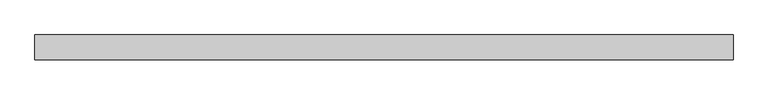
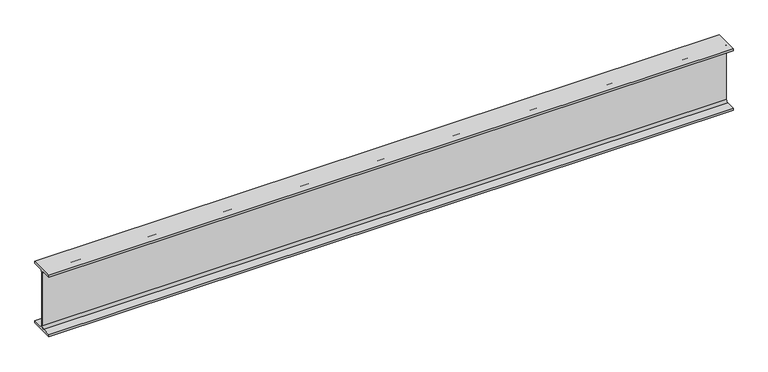
"""IFC4 building model written with IfcOpenShell, lengths in millimetres: beam geometry, 0912_Steel Framing_H-KSD3502 : H_SB_ASB_H-800x300x14x26."""

import ifcopenshell
import ifcopenshell.guid

model = None  # the IFC model being written
_history = None  # IfcOwnerHistory: only IFC2X3 demands one
_inside = {}  # id of a spatial element -> (the spatial element, [elements in it])
_under = {}  # id of a project, library or spatial element -> (it, [spatial elements below it])
_declared = {}  # id of a project -> (the project, [libraries it declares])
_typed = {}  # id of a type object -> (the type object, [elements of that type])
_made_of = {}  # id of a material, layer set ... -> (it, [elements and type objects made of it])


def new_model(schema):
    """Start an empty IFC model of exactly this schema.

    Asked for "IFC4X3", IfcOpenShell would pick the latest addendum, in which some entities
    have other attributes; the version numbers below select the first issue.
    IFC2X3 requires an IfcOwnerHistory on every rooted entity: one is made here for all.
    """
    global model, _history
    if schema == "IFC4X3":
        model = ifcopenshell.file(schema_version=(4, 3, 0, 0))
    else:
        model = ifcopenshell.file(schema=schema)
    _inside.clear()
    _under.clear()
    _declared.clear()
    _typed.clear()
    _made_of.clear()
    _history = None
    if model.schema == "IFC2X3":
        org = make("IfcOrganization", Name="unknown")
        user = make(
            "IfcPersonAndOrganization",
            ThePerson=make("IfcPerson", FamilyName="unknown"),
            TheOrganization=org,
        )
        app = make(
            "IfcApplication",
            ApplicationDeveloper=org,
            Version="unknown",
            ApplicationFullName="unknown",
            ApplicationIdentifier="unknown",
        )
        _history = make(
            "IfcOwnerHistory",
            OwningUser=user,
            OwningApplication=app,
            ChangeAction="ADDED",
            CreationDate=0,
        )
    return model


def make(cls, **values):
    """One entity of the class cls with the attributes given. An attribute that is None is left unset."""
    return model.create_entity(
        cls, **{name: value for name, value in values.items() if value is not None}
    )


def rooted(cls, **values):
    """An entity with a GlobalId (a new one), such as an element, a storey or a relation."""
    return make(cls, GlobalId=ifcopenshell.guid.new(), OwnerHistory=_history, **values)


def si_unit(unit_type, name, prefix=None):
    """IfcSIUnit, for example si_unit("LENGTHUNIT", "METRE", prefix="MILLI")."""
    return make("IfcSIUnit", UnitType=unit_type, Prefix=prefix, Name=name)


def assignment(units):
    """IfcUnitAssignment: the units of a project."""
    return None if units is None else make("IfcUnitAssignment", Units=units)


def point(xyz):
    """IfcCartesianPoint."""
    return None if xyz is None else make("IfcCartesianPoint", Coordinates=xyz)


def direction(xyz):
    """IfcDirection."""
    return None if xyz is None else make("IfcDirection", DirectionRatios=xyz)


def frame(location, z_axis=None, x_axis=None):
    """IfcAxis2Placement3D, a coordinate frame: its origin and axes. An axis left out is left unset."""
    return make(
        "IfcAxis2Placement3D",
        Location=point(location),
        Axis=direction(z_axis),
        RefDirection=direction(x_axis),
    )


def frame_2d(location, x_axis=None):
    """IfcAxis2Placement2D, a coordinate frame in the plane: its origin and x axis."""
    return make(
        "IfcAxis2Placement2D", Location=point(location), RefDirection=direction(x_axis)
    )


def origin():
    """The frame at (0, 0, 0) with its axes left unset."""
    return frame((0.0, 0.0, 0.0))


def place(relative_to, where):
    """IfcLocalPlacement: puts the frame where relative to a parent placement (None: the world)."""
    return make(
        "IfcLocalPlacement", PlacementRelTo=relative_to, RelativePlacement=where
    )


def context(
    kind, dimensions, precision=None, world=None, true_north=None, identifier=None
):
    """IfcGeometricRepresentationContext, for example the 3D "Model" context."""
    return make(
        "IfcGeometricRepresentationContext",
        ContextIdentifier=identifier,
        ContextType=kind,
        CoordinateSpaceDimension=dimensions,
        Precision=precision,
        WorldCoordinateSystem=world,
        TrueNorth=true_north,
    )


def project(units=None, contexts=None):
    """IfcProject with its units and contexts."""
    return rooted(
        "IfcProject",
        Name="project",
        RepresentationContexts=contexts,
        UnitsInContext=assignment(units),
    )


def spatial(cls, under=None, at=None, **own):
    """A site, building, storey or space (cls), placed at a placement, below another one or the project."""
    s = rooted(cls, ObjectPlacement=at, **own)
    if under is not None:
        _under.setdefault(under.id(), (under, []))[1].append(s)
    return s


def polyline(points):
    """IfcPolyline through the points."""
    return make("IfcPolyline", Points=[point(p) for p in points])


def circle_curve(where, radius):
    """IfcCircle in the frame where."""
    return make("IfcCircle", Position=where, Radius=radius)


def trimmed(basis, trim1, trim2, sense, master):
    """IfcTrimmedCurve: the piece of a basis curve between two trims."""
    return make(
        "IfcTrimmedCurve",
        BasisCurve=basis,
        Trim1=trim1,
        Trim2=trim2,
        SenseAgreement=sense,
        MasterRepresentation=master,
    )


def segment(curve, same_sense, transition):
    """IfcCompositeCurveSegment."""
    return make(
        "IfcCompositeCurveSegment",
        Transition=transition,
        SameSense=same_sense,
        ParentCurve=curve,
    )


def composite_curve(segments, self_intersect=None):
    """IfcCompositeCurve: segments joined end to end."""
    return make("IfcCompositeCurve", Segments=segments, SelfIntersect=self_intersect)


def outline(outer, holes=None, kind="AREA"):
    """IfcArbitraryClosedProfileDef: a profile drawn as a closed curve; with holes, ...WithVoids."""
    if holes is None:
        return make("IfcArbitraryClosedProfileDef", ProfileType=kind, OuterCurve=outer)
    return make(
        "IfcArbitraryProfileDefWithVoids",
        ProfileType=kind,
        OuterCurve=outer,
        InnerCurves=holes,
    )


def extrude(swept, where, along, depth):
    """IfcExtrudedAreaSolid: the profile swept, set in the frame where, extruded along a direction by depth."""
    return make(
        "IfcExtrudedAreaSolid",
        SweptArea=swept,
        Position=where,
        ExtrudedDirection=direction(along),
        Depth=depth,
    )


def shape(context_of_items, identifier, shape_type, items):
    """IfcShapeRepresentation: the items that make up one representation, for example the "Body"."""
    return make(
        "IfcShapeRepresentation",
        ContextOfItems=context_of_items,
        RepresentationIdentifier=identifier,
        RepresentationType=shape_type,
        Items=items,
    )


def source(mapping_origin, context_of_items, identifier, shape_type, items):
    """IfcRepresentationMap: a shape defined once, which mapped items show again and again."""
    return make(
        "IfcRepresentationMap",
        MappingOrigin=mapping_origin,
        MappedRepresentation=shape(context_of_items, identifier, shape_type, items),
    )


def transform(
    local_origin,
    x_axis=None,
    y_axis=None,
    z_axis=None,
    scale=None,
    scale2=None,
    scale3=None,
    uniform=True,
):
    """IfcCartesianTransformationOperator3D, or its non-uniform kind. x_axis, y_axis, z_axis: its Axis1, 2, 3."""
    if uniform:
        return make(
            "IfcCartesianTransformationOperator3D",
            Axis1=direction(x_axis),
            Axis2=direction(y_axis),
            LocalOrigin=point(local_origin),
            Scale=scale,
            Axis3=direction(z_axis),
        )
    return make(
        "IfcCartesianTransformationOperator3DnonUniform",
        Axis1=direction(x_axis),
        Axis2=direction(y_axis),
        LocalOrigin=point(local_origin),
        Scale=scale,
        Axis3=direction(z_axis),
        Scale2=scale2,
        Scale3=scale3,
    )


def mapped(mapping_source, mapping_target):
    """IfcMappedItem: shows the shape of a source again, moved by a transform."""
    return make(
        "IfcMappedItem", MappingSource=mapping_source, MappingTarget=mapping_target
    )


def made_of(thing, what):
    """Note that an element or type object is made of a material, layer set ...; save() writes the relation."""
    if what is not None:
        _made_of.setdefault(what.id(), (what, []))[1].append(thing)
    return thing


def element(
    cls,
    number,
    at=None,
    inside=None,
    cuts=None,
    type_object=None,
    material=None,
    context=None,
    identifier="Body",
    shape_type=None,
    held_by="IfcProductDefinitionShape",
    body=None,
    shapes=None,
    **own,
):
    """One element of the class cls, such as IfcWall. Its Tag is "e" and its number.

    at: its placement. inside: the storey or other place that contains it. cuts: it is an
    opening in that element (IfcRelVoidsElement). A single representation is given by context,
    identifier, shape_type and body (its items); several are given by shapes. held_by: the class
    of the entity that holds the representations. save() writes the other relations.
    """
    e = rooted(cls, Tag="e%d" % number, ObjectPlacement=at, **own)
    if body is not None:
        shapes = [shape(context, identifier, shape_type, body)]
    if shapes is not None:
        e.Representation = make(held_by, Representations=shapes)
    if inside is not None:
        _inside.setdefault(inside.id(), (inside, []))[1].append(e)
    if cuts is not None:
        rooted(
            "IfcRelVoidsElement", RelatingBuildingElement=cuts, RelatedOpeningElement=e
        )
    if type_object is not None:
        _typed.setdefault(type_object.id(), (type_object, []))[1].append(e)
    return made_of(e, material)


def aggregate(whole, parts):
    """IfcRelAggregates: a whole, such as a stair, and the parts it consists of."""
    return rooted("IfcRelAggregates", RelatingObject=whole, RelatedObjects=parts)


def save(model, path):
    """Write the relations noted so far, then the file.

    IfcRelAggregates (storeys below a building ...), IfcRelContainedInSpatialStructure (elements
    in a storey), IfcRelDefinesByType, IfcRelAssociatesMaterial and IfcRelDeclares: one each for
    every whole, place, type object, material and project.
    """
    for whole, parts in _under.values():
        aggregate(whole, parts)
    for where, things in _inside.values():
        rooted(
            "IfcRelContainedInSpatialStructure",
            RelatedElements=things,
            RelatingStructure=where,
        )
    for kind, things in _typed.values():
        rooted("IfcRelDefinesByType", RelatedObjects=things, RelatingType=kind)
    for what, things in _made_of.values():
        rooted("IfcRelAssociatesMaterial", RelatedObjects=things, RelatingMaterial=what)
    for by, libraries in _declared.values():
        rooted("IfcRelDeclares", RelatingContext=by, RelatedDefinitions=libraries)
    model.write(path)


def beam_5523baa4(model_context):
    return source(origin(), model_context, "Body", "SweptSolid", [
        extrude(outline(composite_curve([segment(polyline([(150.0, -374.0), (150.0, -400.0), (-150.0, -400.0), (-150.0, -374.0), (-35.0, -374.0)]), True, "CONTINUOUS"), segment(trimmed(circle_curve(frame_2d((-35.0, -346.0)), 28.0), [point((-35.0, -374.0))], [point((-7.0, -346.0))], True, "CARTESIAN"), True, "CONTINUOUS"), segment(polyline([(-7.0, -346.0), (-7.0, 346.0)]), True, "CONTINUOUS"), segment(trimmed(circle_curve(frame_2d((-35.0, 346.0)), 28.0), [point((-7.0, 346.0))], [point((-35.0, 374.0))], True, "CARTESIAN"), True, "CONTINUOUS"), segment(polyline([(-35.0, 374.0), (-150.0, 374.0), (-150.0, 400.0), (150.0, 400.0), (150.0, 374.0), (35.0, 374.0)]), True, "CONTINUOUS"), segment(trimmed(circle_curve(frame_2d((35.0, 346.0)), 28.0), [point((35.0, 374.0))], [point((7.0, 346.0))], True, "CARTESIAN"), True, "CONTINUOUS"), segment(polyline([(7.0, 346.0), (7.0, -346.0)]), True, "CONTINUOUS"), segment(trimmed(circle_curve(frame_2d((35.0, -346.0)), 28.0), [point((7.0, -346.0))], [point((35.0, -374.0))], True, "CARTESIAN"), True, "CONTINUOUS"), segment(polyline([(35.0, -374.0), (150.0, -374.0)]), True, "CONTINUOUS")], self_intersect=False)), frame((-4285.8606617, 0.0, 0.0), z_axis=(1.0, 0.0, 0.0), x_axis=(0.0, 1.0, 0.0)), (0.0, 0.0, 1.0), 8443.8590445),
    ])


if __name__ == "__main__":
    model = new_model("IFC4")
    model_context = context("Model", 3, world=origin())
    ifc_project = project(units=[si_unit("LENGTHUNIT", "METRE", prefix="MILLI")], contexts=[model_context])
    site = spatial("IfcSite", under=ifc_project)
    building = spatial("IfcBuilding", under=site)
    placement = place(None, origin())
    beam_shape = beam_5523baa4(model_context)
    element("IfcBeam", 1, ObjectType="0912_Steel Framing_H-KSD3502 : H_SB_ASB_H-800x300x14x26", at=placement, inside=building, context=model_context, shape_type="MappedRepresentation", body=[
        mapped(beam_shape, transform((0.0, 0.0, 0.0), x_axis=(1.0, 0.0, 0.0), y_axis=(0.0, 1.0, 0.0), z_axis=(0.0, 0.0, 1.0))),
    ])
    save(model, "model.ifc")

# Revit data of these elements
# Type "0912_Steel Framing_H-KSD3502 : H_SB_ASB_H-800x300x14x26"
#   H_WM Code_1 = "S01AA001-00001 | Main Steel Structure Fabrication Work | Shelter/Building | Heavy Steel - Standard (Weight≥90KG/M) | Material: (   )"
#   H_WM Code_2 = "S03AA027-00001 | Main Steel Structure Erection Work | Shelter/Building | Heavy Steel (Weight≥90KG/M) | Material: (   )"
#   H_WM Code_3 = "S01AA010-00001 | Main Steel Structure Fabrication Work | Shelter/Building | Steel Painting/Coating | for Non-Fireproofed Steel Surface, Surface Preparation, Primer, Second & Final Coat | Material: (   )"
#   H_Q'ty Cal Type Tag = "SB-Q2"
#   Width = 30.0 cm
#   Web Thickness = 1.4 cm
#   Web Fillet = 2.8 cm
#   Warping Constant = 17500000.0 cm⁶
#   W = 0
#   Torsional Moment of Inertia = 422.315 cm⁴
#   Section Area = 267.4 cm²
#   Plastic Modulus weak axis = 1220.0 cm³
#   Plastic Modulus strong axis = 8240.0 cm³
#   Perimeter = 2.72 m²/m
#   Nominal Weight = 210.00 kgf/m
#   Moment of Inertia weak axis = 11700.00 cm⁴
#   Moment of Inertia strong axis = 292000.00 cm⁴
#   Height = 80.0 cm
#   Flange Thickness = 2.6 cm
#   Elastic Modulus weak axis = 782.0 cm³
#   Elastic Modulus strong axis = 7290.0 cm³
#   Centroid Vertical = 40.0 cm
#   Centroid Horizontal = 15.0 cm
#   Ix = 2920000000
#   Length [instance default] = 1.5240 m
#   Zx = 8240000
#   b = 0.3000 m
#   h = 0.8000 m
#   r = 0.0280 m
#   s = 0.0140 m
#   t = 0.0260 m
#   A = 0.02674 m²
#   Structural Material [instance default] = Steel, 45-345
#   Assembly Code = ""
# Element 1 (IfcBeam, "0912_Steel Framing_H-KSD3502 : H_SB_ASB_H-800x300x14x26")
#   Structural Material = none
# Materials
#   "Steel, 45-345": class "Metal", colour RGB 189 187 185, transparency 0, Description = "Steel 345 MPa", Cost = 0
